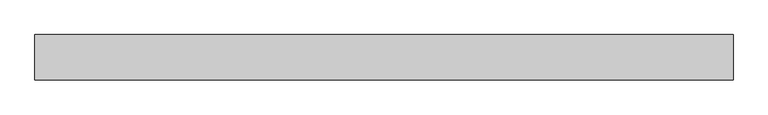
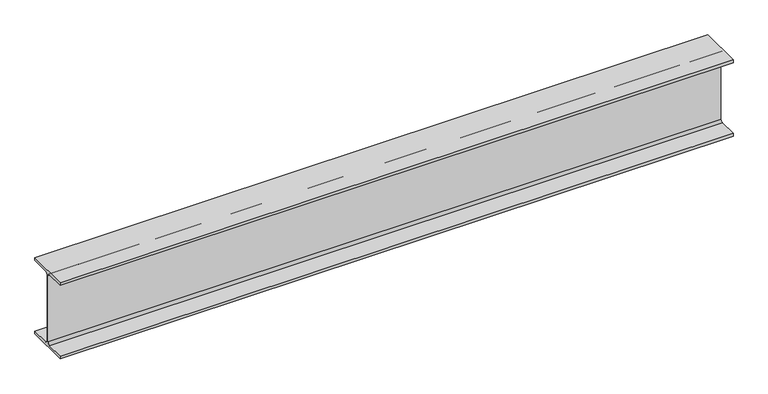
"""IFC4 building model written with IfcOpenShell, lengths in millimetres: beam geometry, Old_Steel Beam_H-KSD3502 : H_SB_ASB_H-350×175x7x11."""

from ifc_helpers import new_model, si_unit, point, frame, frame_2d, origin, place, context, project, spatial, polyline, circle_curve, trimmed, segment, composite_curve, outline, extrude, source, transform, mapped, element, save


def beam_2392fa11(model_context):
    return source(origin(), model_context, "Body", "SweptSolid", [
        extrude(outline(composite_curve([segment(polyline([(82.5, -141.5), (82.5, -151.7), (-82.5, -151.7), (-82.5, -141.5), (-11.9, -141.5)]), True, "CONTINUOUS"), segment(trimmed(circle_curve(frame_2d((-11.9, -132.6)), 8.9), [point((-11.9, -141.5))], [point((-3.0, -132.6))], True, "CARTESIAN"), True, "CONTINUOUS"), segment(polyline([(-3.0, -132.6), (-3.0, 132.6)]), True, "CONTINUOUS"), segment(trimmed(circle_curve(frame_2d((-11.9, 132.6)), 8.9), [point((-3.0, 132.6))], [point((-11.9, 141.5))], True, "CARTESIAN"), True, "CONTINUOUS"), segment(polyline([(-11.9, 141.5), (-82.5, 141.5), (-82.5, 151.7), (82.5, 151.7), (82.5, 141.5), (11.9, 141.5)]), True, "CONTINUOUS"), segment(trimmed(circle_curve(frame_2d((11.9, 132.6)), 8.9), [point((11.9, 141.5))], [point((3.0, 132.6))], True, "CARTESIAN"), True, "CONTINUOUS"), segment(polyline([(3.0, 132.6), (3.0, -132.6)]), True, "CONTINUOUS"), segment(trimmed(circle_curve(frame_2d((11.9, -132.6)), 8.9), [point((3.0, -132.6))], [point((11.9, -141.5))], True, "CARTESIAN"), True, "CONTINUOUS"), segment(polyline([(11.9, -141.5), (82.5, -141.5)]), True, "CONTINUOUS")], self_intersect=False)), frame((-1295.7739051, 0.0, 0.0), z_axis=(1.0, 0.0, 0.0), x_axis=(0.0, 1.0, 0.0)), (0.0, 0.0, 1.0), 2540.0189947),
    ])


if __name__ == "__main__":
    model = new_model("IFC4")
    model_context = context("Model", 3, world=origin())
    ifc_project = project(units=[si_unit("LENGTHUNIT", "METRE", prefix="MILLI")], contexts=[model_context])
    site = spatial("IfcSite", under=ifc_project)
    building = spatial("IfcBuilding", under=site)
    placement = place(None, origin())
    beam_shape = beam_2392fa11(model_context)
    element("IfcBeam", 1, ObjectType="Old_Steel Beam_H-KSD3502 : H_SB_ASB_H-350×175x7x11", at=placement, inside=building, context=model_context, shape_type="MappedRepresentation", body=[
        mapped(beam_shape, transform((0.0, 0.0, 0.0), x_axis=(1.0, 0.0, 0.0), y_axis=(0.0, 1.0, 0.0), z_axis=(0.0, 0.0, 1.0))),
    ])
    save(model, "model.ifc")

# Revit data of these elements
# Type "Old_Steel Beam_H-KSD3502 : H_SB_ASB_H-350×175x7x11"
#   Width = 17.5 cm
#   Web Thickness = 0.7 cm
#   Web Fillet = 1.4 cm
#   Warping Constant = 282290.0 cm⁶
#   Torsional Moment of Inertia = 19.4042 cm⁴
#   Torsional Modulus = 1.0 cm³
#   Section Area = 63.14 cm²
#   Plastic Modulus weak axis = 174.0 cm³
#   Plastic Modulus strong axis = 868.0 cm³
#   Perimeter = 1.36 m²/m
#   Nominal Weight = 49.60 kgf/m
#   Moment of Inertia weak axis = 984.00 cm⁴
#   Moment of Inertia strong axis = 13600.00 cm⁴
#   Height = 35.0 cm
#   Flange Thickness = 1.1 cm
#   Elastic Modulus weak axis = 112.0 cm³
#   Elastic Modulus strong axis = 775.0 cm³
#   Centroid Vertical = 17.5 cm
#   Centroid Horizontal = 8.75 cm
#   Length [instance default] = 1.5240 m
#   Structural Material [instance default] = Steel, 45-345
#   Assembly Code = ""
# Element 1 (IfcBeam, "Old_Steel Beam_H-KSD3502 : H_SB_ASB_H-350×175x7x11")
#   Structural Material = none
# Materials
#   "Steel, 45-345": class "Metal", colour RGB 189 187 185, transparency 0, Description = "Steel 345 MPa", Cost = 0
